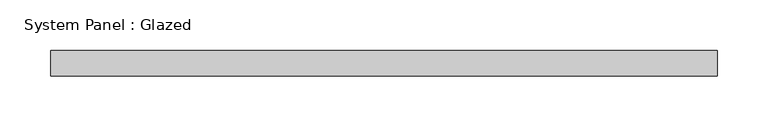
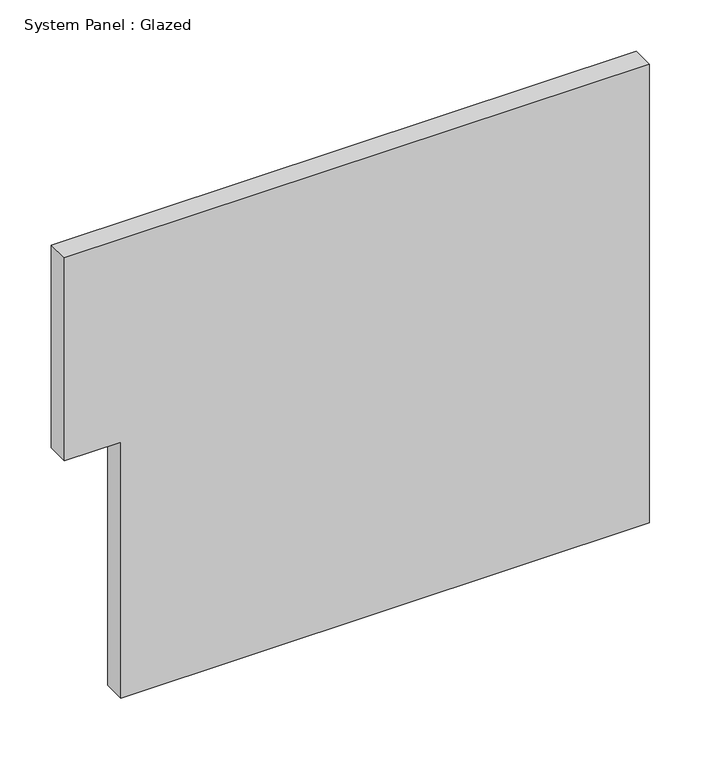
"""IFC4 building model written with IfcOpenShell, lengths in millimetres: plate geometry, System Panel : Glazed."""

from ifc_helpers import new_model, si_unit, frame, origin, place, context, project, spatial, polyline, outline, extrude, source, transform, mapped, element, save


def system_panel_glazed_78103c7b(model_context):
    return source(origin(), model_context, "Body", "SweptSolid", [
        extrude(outline(polyline([(0.0, -265.95), (0.0, 329.45), (304.8, 329.45), (546.1, 329.45), (546.1, -329.45), (304.8, -329.45), (304.8, -265.95), (0.0, -265.95)])), frame((0.0, -44.45, 0.0), z_axis=(0.0, 1.0, 0.0), x_axis=(0.0, 0.0, 1.0)), (0.0, 0.0, 1.0), 25.4),
    ])


if __name__ == "__main__":
    model = new_model("IFC4")
    model_context = context("Model", 3, world=origin())
    ifc_project = project(units=[si_unit("LENGTHUNIT", "METRE", prefix="MILLI")], contexts=[model_context])
    site = spatial("IfcSite", under=ifc_project)
    building = spatial("IfcBuilding", under=site)
    placement = place(None, origin())
    system_panel_glazed_shape = system_panel_glazed_78103c7b(model_context)
    element("IfcPlate", 1, ObjectType="System Panel : Glazed", at=placement, inside=building, context=model_context, shape_type="MappedRepresentation", body=[
        mapped(system_panel_glazed_shape, transform((0.0, 0.0, 0.0), x_axis=(1.0, 0.0, 0.0), y_axis=(0.0, 1.0, 0.0), z_axis=(0.0, 0.0, 1.0))),
    ])
    save(model, "model.ifc")

# Revit data of these elements
# Element 1 (IfcPlate, "System Panel : Glazed")
#   Materials on its faces: "Glass"
# Materials
#   "Glass": class "Glass", colour RGB 0 128 192, transparency 0.75, Cost = 0
